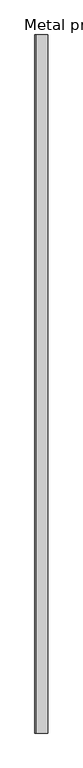
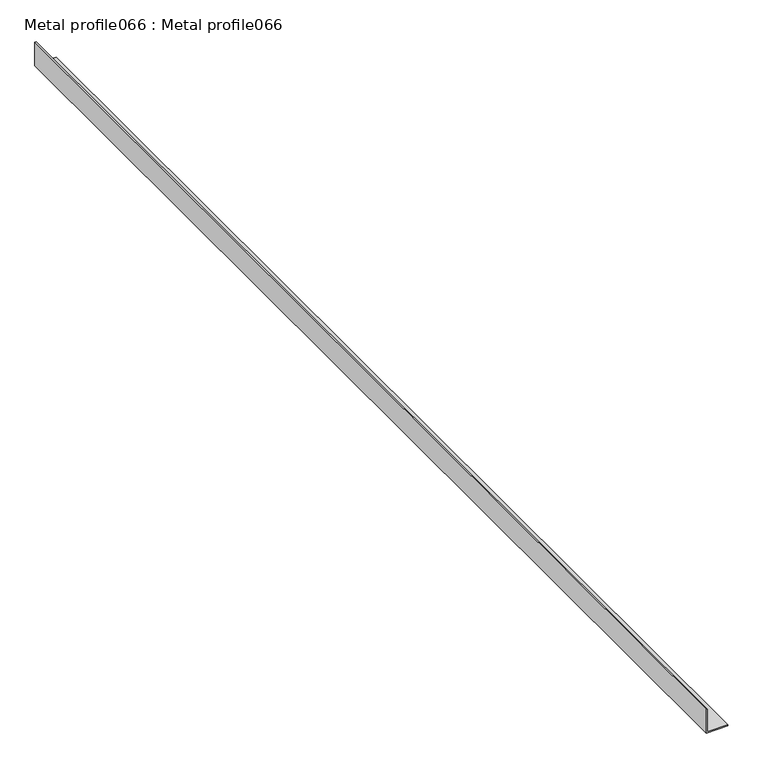
"""IFC4 building model written with IfcOpenShell, lengths in millimetres: proxy geometry, Metal profile066 : Metal profile066."""

from ifc_helpers import new_model, si_unit, frame, origin, place, context, project, spatial, polyline, outline, extrude, source, transform, mapped, element, save


def metal_profile066_metal_profile066_326c48cf(model_context):
    return source(origin(), model_context, "Body", "SweptSolid", [
        extrude(outline(polyline([(36439.5390625, -6024.875), (36439.5390625, -6059.8710938), (36480.4296875, -6059.8710938), (36480.4296875, -6061.8710937), (36437.5390625, -6061.8710937), (36437.5390625, -6024.875), (36439.5390625, -6024.875)])), frame((0.0, -1052.8906574, 0.0), z_axis=(0.0, 1.0, 0.0), x_axis=(0.0, 0.0, 1.0)), (0.0, 0.0, 1.0), 2000.0),
    ])


if __name__ == "__main__":
    model = new_model("IFC4")
    model_context = context("Model", 3, world=origin())
    ifc_project = project(units=[si_unit("LENGTHUNIT", "METRE", prefix="MILLI")], contexts=[model_context])
    site = spatial("IfcSite", under=ifc_project)
    building = spatial("IfcBuilding", under=site)
    placement = place(None, origin())
    metal_profile066_metal_profile066_shape = metal_profile066_metal_profile066_326c48cf(model_context)
    element("IfcBuildingElementProxy", 1, Name="Metal profile066 : Metal profile066", ObjectType="Metal profile066 : Metal profile066", at=placement, inside=building, context=model_context, shape_type="MappedRepresentation", body=[
        mapped(metal_profile066_metal_profile066_shape, transform((0.0, 0.0, 0.0), x_axis=(1.0, 0.0, 0.0), y_axis=(0.0, 1.0, 0.0), z_axis=(0.0, 0.0, 1.0))),
    ])
    save(model, "model.ifc")

# Revit data of these elements
# Type "Metal profile066 : Metal profile066"
#   NameOverride = "Metal profile066"
# Element 1 (IfcBuildingElementProxy, "Metal profile066 : Metal profile066")
#   Materials on its faces: "L-SHAPED METAL TRIM"
# Materials
#   "L-SHAPED METAL TRIM": class "Unassigned", colour RGB 255 231 0, transparency 0
